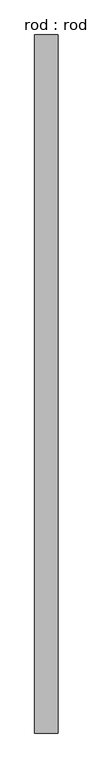
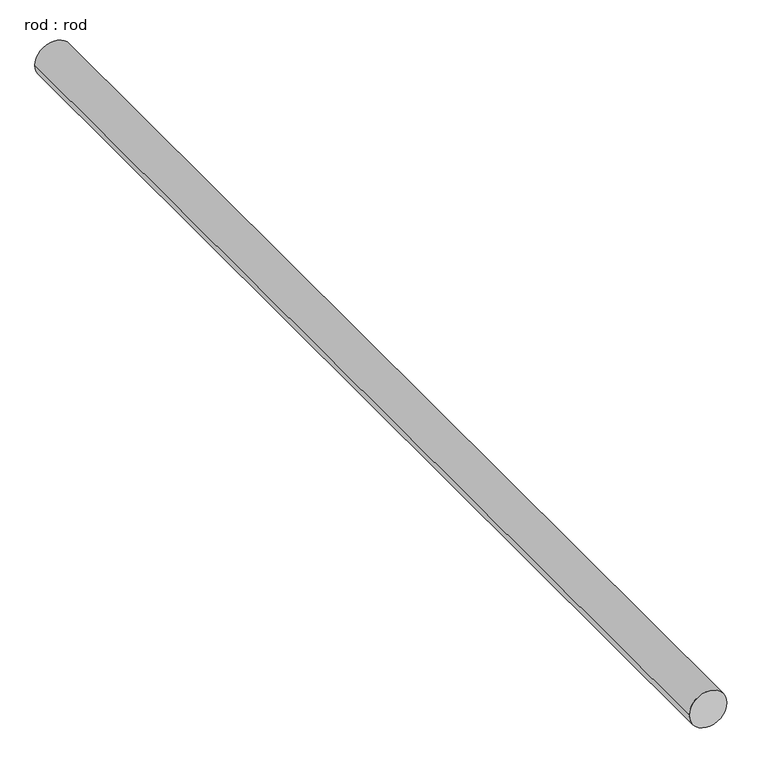
"""IFC4 building model written with IfcOpenShell, lengths in millimetres: proxy geometry, rod : rod."""

import ifcopenshell
import ifcopenshell.guid

model = None  # the IFC model being written
_history = None  # IfcOwnerHistory: only IFC2X3 demands one
_inside = {}  # id of a spatial element -> (the spatial element, [elements in it])
_under = {}  # id of a project, library or spatial element -> (it, [spatial elements below it])
_declared = {}  # id of a project -> (the project, [libraries it declares])
_typed = {}  # id of a type object -> (the type object, [elements of that type])
_made_of = {}  # id of a material, layer set ... -> (it, [elements and type objects made of it])


def new_model(schema):
    """Start an empty IFC model of exactly this schema.

    Asked for "IFC4X3", IfcOpenShell would pick the latest addendum, in which some entities
    have other attributes; the version numbers below select the first issue.
    IFC2X3 requires an IfcOwnerHistory on every rooted entity: one is made here for all.
    """
    global model, _history
    if schema == "IFC4X3":
        model = ifcopenshell.file(schema_version=(4, 3, 0, 0))
    else:
        model = ifcopenshell.file(schema=schema)
    _inside.clear()
    _under.clear()
    _declared.clear()
    _typed.clear()
    _made_of.clear()
    _history = None
    if model.schema == "IFC2X3":
        org = make("IfcOrganization", Name="unknown")
        user = make(
            "IfcPersonAndOrganization",
            ThePerson=make("IfcPerson", FamilyName="unknown"),
            TheOrganization=org,
        )
        app = make(
            "IfcApplication",
            ApplicationDeveloper=org,
            Version="unknown",
            ApplicationFullName="unknown",
            ApplicationIdentifier="unknown",
        )
        _history = make(
            "IfcOwnerHistory",
            OwningUser=user,
            OwningApplication=app,
            ChangeAction="ADDED",
            CreationDate=0,
        )
    return model


def make(cls, **values):
    """One entity of the class cls with the attributes given. An attribute that is None is left unset."""
    return model.create_entity(
        cls, **{name: value for name, value in values.items() if value is not None}
    )


def rooted(cls, **values):
    """An entity with a GlobalId (a new one), such as an element, a storey or a relation."""
    return make(cls, GlobalId=ifcopenshell.guid.new(), OwnerHistory=_history, **values)


def si_unit(unit_type, name, prefix=None):
    """IfcSIUnit, for example si_unit("LENGTHUNIT", "METRE", prefix="MILLI")."""
    return make("IfcSIUnit", UnitType=unit_type, Prefix=prefix, Name=name)


def assignment(units):
    """IfcUnitAssignment: the units of a project."""
    return None if units is None else make("IfcUnitAssignment", Units=units)


def point(xyz):
    """IfcCartesianPoint."""
    return None if xyz is None else make("IfcCartesianPoint", Coordinates=xyz)


def direction(xyz):
    """IfcDirection."""
    return None if xyz is None else make("IfcDirection", DirectionRatios=xyz)


def frame(location, z_axis=None, x_axis=None):
    """IfcAxis2Placement3D, a coordinate frame: its origin and axes. An axis left out is left unset."""
    return make(
        "IfcAxis2Placement3D",
        Location=point(location),
        Axis=direction(z_axis),
        RefDirection=direction(x_axis),
    )


def frame_2d(location, x_axis=None):
    """IfcAxis2Placement2D, a coordinate frame in the plane: its origin and x axis."""
    return make(
        "IfcAxis2Placement2D", Location=point(location), RefDirection=direction(x_axis)
    )


def origin():
    """The frame at (0, 0, 0) with its axes left unset."""
    return frame((0.0, 0.0, 0.0))


def place(relative_to, where):
    """IfcLocalPlacement: puts the frame where relative to a parent placement (None: the world)."""
    return make(
        "IfcLocalPlacement", PlacementRelTo=relative_to, RelativePlacement=where
    )


def context(
    kind, dimensions, precision=None, world=None, true_north=None, identifier=None
):
    """IfcGeometricRepresentationContext, for example the 3D "Model" context."""
    return make(
        "IfcGeometricRepresentationContext",
        ContextIdentifier=identifier,
        ContextType=kind,
        CoordinateSpaceDimension=dimensions,
        Precision=precision,
        WorldCoordinateSystem=world,
        TrueNorth=true_north,
    )


def project(units=None, contexts=None):
    """IfcProject with its units and contexts."""
    return rooted(
        "IfcProject",
        Name="project",
        RepresentationContexts=contexts,
        UnitsInContext=assignment(units),
    )


def spatial(cls, under=None, at=None, **own):
    """A site, building, storey or space (cls), placed at a placement, below another one or the project."""
    s = rooted(cls, ObjectPlacement=at, **own)
    if under is not None:
        _under.setdefault(under.id(), (under, []))[1].append(s)
    return s


def circle_curve(where, radius):
    """IfcCircle in the frame where."""
    return make("IfcCircle", Position=where, Radius=radius)


def trimmed(basis, trim1, trim2, sense, master):
    """IfcTrimmedCurve: the piece of a basis curve between two trims."""
    return make(
        "IfcTrimmedCurve",
        BasisCurve=basis,
        Trim1=trim1,
        Trim2=trim2,
        SenseAgreement=sense,
        MasterRepresentation=master,
    )


def segment(curve, same_sense, transition):
    """IfcCompositeCurveSegment."""
    return make(
        "IfcCompositeCurveSegment",
        Transition=transition,
        SameSense=same_sense,
        ParentCurve=curve,
    )


def composite_curve(segments, self_intersect=None):
    """IfcCompositeCurve: segments joined end to end."""
    return make("IfcCompositeCurve", Segments=segments, SelfIntersect=self_intersect)


def outline(outer, holes=None, kind="AREA"):
    """IfcArbitraryClosedProfileDef: a profile drawn as a closed curve; with holes, ...WithVoids."""
    if holes is None:
        return make("IfcArbitraryClosedProfileDef", ProfileType=kind, OuterCurve=outer)
    return make(
        "IfcArbitraryProfileDefWithVoids",
        ProfileType=kind,
        OuterCurve=outer,
        InnerCurves=holes,
    )


def extrude(swept, where, along, depth):
    """IfcExtrudedAreaSolid: the profile swept, set in the frame where, extruded along a direction by depth."""
    return make(
        "IfcExtrudedAreaSolid",
        SweptArea=swept,
        Position=where,
        ExtrudedDirection=direction(along),
        Depth=depth,
    )


def shape(context_of_items, identifier, shape_type, items):
    """IfcShapeRepresentation: the items that make up one representation, for example the "Body"."""
    return make(
        "IfcShapeRepresentation",
        ContextOfItems=context_of_items,
        RepresentationIdentifier=identifier,
        RepresentationType=shape_type,
        Items=items,
    )


def source(mapping_origin, context_of_items, identifier, shape_type, items):
    """IfcRepresentationMap: a shape defined once, which mapped items show again and again."""
    return make(
        "IfcRepresentationMap",
        MappingOrigin=mapping_origin,
        MappedRepresentation=shape(context_of_items, identifier, shape_type, items),
    )


def transform(
    local_origin,
    x_axis=None,
    y_axis=None,
    z_axis=None,
    scale=None,
    scale2=None,
    scale3=None,
    uniform=True,
):
    """IfcCartesianTransformationOperator3D, or its non-uniform kind. x_axis, y_axis, z_axis: its Axis1, 2, 3."""
    if uniform:
        return make(
            "IfcCartesianTransformationOperator3D",
            Axis1=direction(x_axis),
            Axis2=direction(y_axis),
            LocalOrigin=point(local_origin),
            Scale=scale,
            Axis3=direction(z_axis),
        )
    return make(
        "IfcCartesianTransformationOperator3DnonUniform",
        Axis1=direction(x_axis),
        Axis2=direction(y_axis),
        LocalOrigin=point(local_origin),
        Scale=scale,
        Axis3=direction(z_axis),
        Scale2=scale2,
        Scale3=scale3,
    )


def mapped(mapping_source, mapping_target):
    """IfcMappedItem: shows the shape of a source again, moved by a transform."""
    return make(
        "IfcMappedItem", MappingSource=mapping_source, MappingTarget=mapping_target
    )


def made_of(thing, what):
    """Note that an element or type object is made of a material, layer set ...; save() writes the relation."""
    if what is not None:
        _made_of.setdefault(what.id(), (what, []))[1].append(thing)
    return thing


def element(
    cls,
    number,
    at=None,
    inside=None,
    cuts=None,
    type_object=None,
    material=None,
    context=None,
    identifier="Body",
    shape_type=None,
    held_by="IfcProductDefinitionShape",
    body=None,
    shapes=None,
    **own,
):
    """One element of the class cls, such as IfcWall. Its Tag is "e" and its number.

    at: its placement. inside: the storey or other place that contains it. cuts: it is an
    opening in that element (IfcRelVoidsElement). A single representation is given by context,
    identifier, shape_type and body (its items); several are given by shapes. held_by: the class
    of the entity that holds the representations. save() writes the other relations.
    """
    e = rooted(cls, Tag="e%d" % number, ObjectPlacement=at, **own)
    if body is not None:
        shapes = [shape(context, identifier, shape_type, body)]
    if shapes is not None:
        e.Representation = make(held_by, Representations=shapes)
    if inside is not None:
        _inside.setdefault(inside.id(), (inside, []))[1].append(e)
    if cuts is not None:
        rooted(
            "IfcRelVoidsElement", RelatingBuildingElement=cuts, RelatedOpeningElement=e
        )
    if type_object is not None:
        _typed.setdefault(type_object.id(), (type_object, []))[1].append(e)
    return made_of(e, material)


def aggregate(whole, parts):
    """IfcRelAggregates: a whole, such as a stair, and the parts it consists of."""
    return rooted("IfcRelAggregates", RelatingObject=whole, RelatedObjects=parts)


def save(model, path):
    """Write the relations noted so far, then the file.

    IfcRelAggregates (storeys below a building ...), IfcRelContainedInSpatialStructure (elements
    in a storey), IfcRelDefinesByType, IfcRelAssociatesMaterial and IfcRelDeclares: one each for
    every whole, place, type object, material and project.
    """
    for whole, parts in _under.values():
        aggregate(whole, parts)
    for where, things in _inside.values():
        rooted(
            "IfcRelContainedInSpatialStructure",
            RelatedElements=things,
            RelatingStructure=where,
        )
    for kind, things in _typed.values():
        rooted("IfcRelDefinesByType", RelatedObjects=things, RelatingType=kind)
    for what, things in _made_of.values():
        rooted("IfcRelAssociatesMaterial", RelatedObjects=things, RelatingMaterial=what)
    for by, libraries in _declared.values():
        rooted("IfcRelDeclares", RelatingContext=by, RelatedDefinitions=libraries)
    model.write(path)


def rod_rod_b4dfb3ef(model_context):
    return source(origin(), model_context, "Body", "SweptSolid", [
        extrude(outline(composite_curve([segment(trimmed(circle_curve(frame_2d((0.0108462, 0.0)), 200.0), [point((0.0108462, 200.0))], [point((0.0108462, -200.0))], False, "CARTESIAN"), True, "CONTINUOUS"), segment(trimmed(circle_curve(frame_2d((0.0108462, 0.0)), 200.0), [point((0.0108462, -200.0))], [point((0.0108462, 200.0))], False, "CARTESIAN"), True, "CONTINUOUS")], self_intersect=False)), frame((0.0, -1908.5537997, 0.0), z_axis=(0.0, 1.0, 0.0), x_axis=(0.0, 0.0, 1.0)), (0.0, 0.0, 1.0), 12002.5648301),
    ])


if __name__ == "__main__":
    model = new_model("IFC4")
    model_context = context("Model", 3, world=origin())
    ifc_project = project(units=[si_unit("LENGTHUNIT", "METRE", prefix="MILLI")], contexts=[model_context])
    site = spatial("IfcSite", under=ifc_project)
    building = spatial("IfcBuilding", under=site)
    placement = place(None, origin())
    rod_rod_shape = rod_rod_b4dfb3ef(model_context)
    element("IfcBuildingElementProxy", 1, Name="rod : rod", ObjectType="rod : rod", at=placement, inside=building, context=model_context, shape_type="MappedRepresentation", body=[
        mapped(rod_rod_shape, transform((0.0, 0.0, 0.0), x_axis=(1.0, 0.0, 0.0), y_axis=(0.0, 1.0, 0.0), z_axis=(0.0, 0.0, 1.0))),
    ])
    save(model, "model.ifc")

# Revit data of these elements
# Type "rod : rod"
#   Default Elevation = 0
